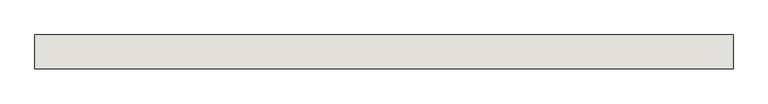
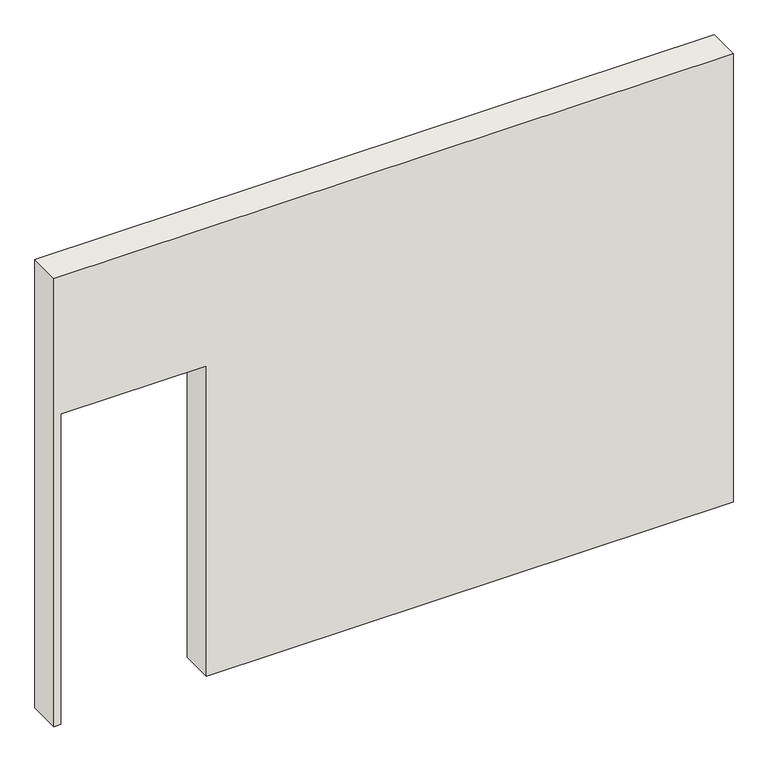
"""IFC4 building model written with IfcOpenShell, lengths in millimetres: wall geometry, Holzwand."""

from ifc_helpers import new_model, si_unit, frame, origin, place, context, project, spatial, polyline, outline, extrude, source, transform, mapped, element, save


def wall_c8f5c598(model_context):
    return source(origin(), model_context, "Body", "SweptSolid", [
        extrude(outline(polyline([(1995.0, 925.9795824), (0.0, 925.9795824), (0.0, 4125.9795824), (2880.0, 4125.9795824), (2880.0, 0.0), (0.0, 0.0), (0.0, 40.9795824), (1995.0, 40.9795824), (1995.0, 925.9795824)])), frame((0.0, 0.0, 0.0), z_axis=(0.0, 1.0, 0.0), x_axis=(0.0, 0.0, 1.0)), (0.0, 0.0, 1.0), 200.0),
    ])


if __name__ == "__main__":
    model = new_model("IFC4")
    model_context = context("Model", 3, world=origin())
    ifc_project = project(units=[si_unit("LENGTHUNIT", "METRE", prefix="MILLI")], contexts=[model_context])
    site = spatial("IfcSite", under=ifc_project)
    building = spatial("IfcBuilding", under=site)
    placement = place(None, origin())
    wall_shape = wall_c8f5c598(model_context)
    element("IfcWall", 1, ObjectType="Holzwand", at=placement, inside=building, context=model_context, shape_type="MappedRepresentation", body=[
        mapped(wall_shape, transform((0.0, 0.0, 0.0), x_axis=(1.0, 0.0, 0.0), y_axis=(0.0, 1.0, 0.0), z_axis=(0.0, 0.0, 1.0))),
    ])
    save(model, "model.ifc")

# Revit data of these elements
# Element 1 (IfcWall, "Holzwand")
#   Materials on its faces: "holzschalung"
# Materials
#   "holzschalung": class "Unassigned", colour RGB 128 128 128, transparency 0
